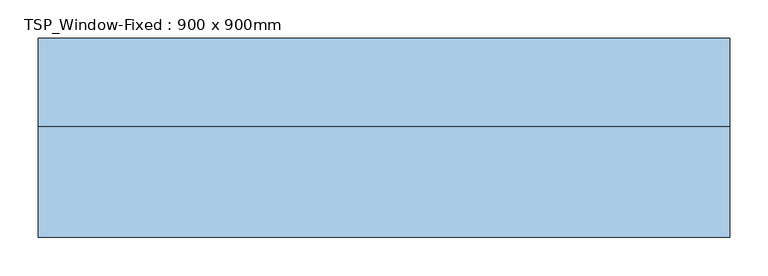
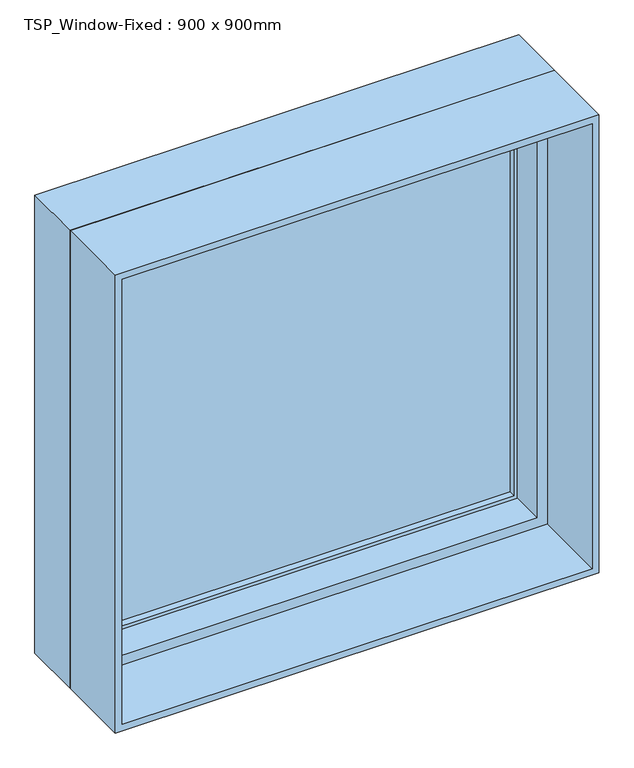
"""IFC4 building model written with IfcOpenShell, lengths in millimetres: window geometry, TSP_Window-Fixed : 900 x 900mm."""

from ifc_helpers import new_model, si_unit, frame, origin, place, context, project, spatial, polyline, outline, extrude, faceted_brep, source, transform, mapped, element, save


def tsp_window_fixed_900_x_900mm_6e251a3b(model_context):
    return source(origin(), model_context, "Body", "SolidModel", [
        faceted_brep([(450.0, 24.75, 1800.0), (450.0, 139.05, 1800.0), (-450.0, 139.05, 1800.0), (-450.0, 24.75, 1800.0), (-450.0, 139.05, 900.0), (-450.0, 24.75, 900.0), (450.0, 139.05, 900.0), (450.0, 24.75, 900.0), (418.25, 24.75, 1768.25), (418.25, 24.75, 931.75), (-418.25, 24.75, 931.75), (-418.25, 24.75, 1768.25), (-437.3, 139.05, 1787.3), (-437.3, 139.05, 912.7), (437.3, 139.05, 912.7), (437.3, 139.05, 1787.3), (418.25, 88.25, 1768.25), (-418.25, 88.25, 1768.25), (437.3, 88.25, 1787.3), (-437.3, 88.25, 1787.3), (-418.25, 88.25, 931.75), (-437.3, 88.25, 912.7), (418.25, 88.25, 931.75), (437.3, 88.25, 912.7)], [[[0, 1, 2, 3]], [[3, 2, 4, 5]], [[5, 4, 6, 7]], [[3, 5, 7, 0], [8, 9, 10, 11]], [[7, 6, 1, 0]], [[1, 6, 4, 2], [12, 13, 14, 15]], [[16, 8, 11, 17]], [[15, 18, 19, 12]], [[17, 11, 10, 20]], [[12, 19, 21, 13]], [[20, 10, 9, 22]], [[13, 21, 23, 14]], [[22, 9, 8, 16]], [[18, 23, 21, 19], [17, 20, 22, 16]], [[14, 23, 18, 15]]]),
        extrude(outline(polyline([(1800.0, -450.0), (900.0, -450.0), (900.0, 450.0), (1800.0, 450.0), (1800.0, -450.0)]), holes=[polyline([(1787.3, 437.3), (912.7, 437.3), (912.7, -437.3), (1787.3, -437.3), (1787.3, 437.3)])]), frame((0.0, -120.0, 0.0), z_axis=(0.0, 1.0, 0.0), x_axis=(0.0, 0.0, 1.0)), (0.0, 0.0, 1.0), 144.75),
        extrude(outline(polyline([(912.7, 437.3), (1787.3, 437.3), (1787.3, -437.3), (912.7, -437.3), (912.7, 437.3)]), holes=[polyline([(938.1, -411.9), (1761.9, -411.9), (1761.9, 411.9), (938.1, 411.9), (938.1, -411.9)])]), frame((0.0, 88.25, 0.0), z_axis=(0.0, 1.0, 0.0), x_axis=(0.0, 0.0, 1.0)), (0.0, 0.0, 1.0), 44.45),
        extrude(outline(polyline([(411.9, 120.0), (411.9, 113.65), (-411.9, 113.65), (-411.9, 120.0), (411.9, 120.0)])), frame((0.0, 0.0, 938.1), z_axis=(0.0, 0.0, 1.0), x_axis=(1.0, 0.0, 0.0)), (0.0, 0.0, 1.0), 823.8),
        extrude(outline(polyline([(-411.9, 100.95), (-411.9, 107.3), (411.9, 107.3), (411.9, 100.95), (-411.9, 100.95)])), frame((0.0, 0.0, 938.1), z_axis=(0.0, 0.0, 1.0), x_axis=(1.0, 0.0, 0.0)), (0.0, 0.0, 1.0), 823.8),
    ])


if __name__ == "__main__":
    model = new_model("IFC4")
    model_context = context("Model", 3, world=origin())
    ifc_project = project(units=[si_unit("LENGTHUNIT", "METRE", prefix="MILLI")], contexts=[model_context])
    site = spatial("IfcSite", under=ifc_project)
    building = spatial("IfcBuilding", under=site)
    placement = place(None, origin())
    tsp_window_fixed_900_x_900mm_shape = tsp_window_fixed_900_x_900mm_6e251a3b(model_context)
    element("IfcWindow", 1, ObjectType="TSP_Window-Fixed : 900 x 900mm", at=placement, inside=building, context=model_context, shape_type="MappedRepresentation", body=[
        mapped(tsp_window_fixed_900_x_900mm_shape, transform((0.0, 0.0, 0.0), x_axis=(1.0, 0.0, 0.0), y_axis=(0.0, 1.0, 0.0), z_axis=(0.0, 0.0, 1.0))),
    ])
    save(model, "model.ifc")

# Revit data of these elements
# Type "TSP_Window-Fixed : 900 x 900mm"
#   Type Mark = "HS 2412 F148"
#   Fire Rating = "0.5h"
#   Assembly Code = "B2020100"
#   Analytic Construction = "Double glazing - domestic"
#   Window Inset [instance default] = 0 mm
#   Wall Thickness [instance default] = 150 mm
#   Visual Light Transmittance = 0.81
#   Thermal Resistance (R) = 0.319569 (m²·K)/W
#   Solar Heat Gain Coefficient = 0.76
#   Rough Width = 915 mm
#   Rough Height = 915 mm
#   Interior Wall Closure [instance default] = 54.75 mm
#   Height = 900 mm
#   Heat Transfer Coefficient (U) = 3.12929 W/(m²·K)
#   Frame Extension [instance default] = 6.35 mm
#   Exterior Wall Closure [instance default] = 31.75 mm
#   Extension Jamb [instance default] = 54.75 mm
#   Default Sill Height = 900 mm
#   Width = 900 mm
#   Muntin Visibility = yes
#   Interior Trim Visibility [instance default] = yes
#   Exterior Trim Visibility [instance default] = yes
#   Extension Jamb Visibility [instance default] = yes
#   Interior Trim Material = Wood - Stained
#   Interior Frame Material = Wood - Stained
#   Glass Panel Material = Glass
#   Exterior Trim Material = Clad - White
#   Exterior Frame Material = Clad - White
#   Wall Closure = (empty or 0)
# Element 1 (IfcWindow, "TSP_Window-Fixed : 900 x 900mm")
#   Wall Thickness = 240 mm
#   Extension Jamb = 144.75 mm
#   Materials on its faces: "Wood - Stained", "Glass", "Clad - White"
# Materials
#   "Wood - Stained": class "Wood", colour RGB 224 178 126, transparency 0, Cost = 0
#   "Glass": class "Glass", colour RGB 0 128 192, transparency 0.9, Description = "Soda Lime Glass", Cost = 0
#   "Clad - White": class "Wood", colour RGB 242 242 238, transparency 0, Cost = 0
